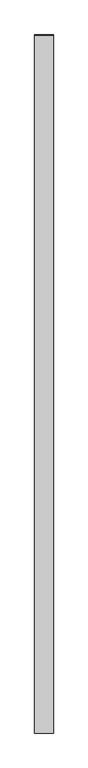
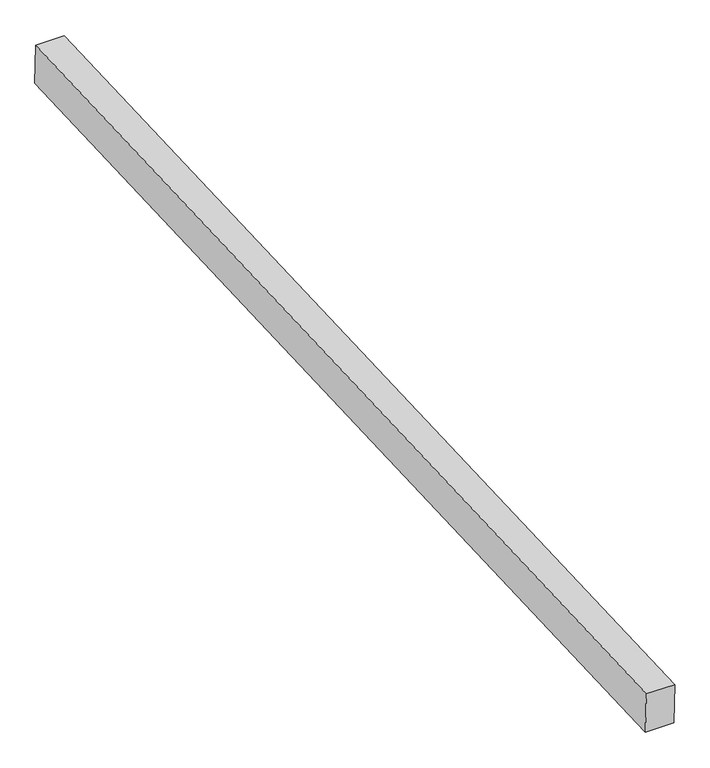
"""IFC4 building model written with IfcOpenShell, lengths in millimetres: proxy geometry, Generic Models 7:Generic Models 1:8:Generic Models 1:8 : Generic Models 7:Generic Models 1:337419:24 : Generic Models 7:Generic Models 1:8:Generic Models 1:8 : Generic Models 7:Generic Models 1:337419:315935."""

import ifcopenshell
import ifcopenshell.guid

model = None  # the IFC model being written
_history = None  # IfcOwnerHistory: only IFC2X3 demands one
_inside = {}  # id of a spatial element -> (the spatial element, [elements in it])
_under = {}  # id of a project, library or spatial element -> (it, [spatial elements below it])
_declared = {}  # id of a project -> (the project, [libraries it declares])
_typed = {}  # id of a type object -> (the type object, [elements of that type])
_made_of = {}  # id of a material, layer set ... -> (it, [elements and type objects made of it])


def new_model(schema):
    """Start an empty IFC model of exactly this schema.

    Asked for "IFC4X3", IfcOpenShell would pick the latest addendum, in which some entities
    have other attributes; the version numbers below select the first issue.
    IFC2X3 requires an IfcOwnerHistory on every rooted entity: one is made here for all.
    """
    global model, _history
    if schema == "IFC4X3":
        model = ifcopenshell.file(schema_version=(4, 3, 0, 0))
    else:
        model = ifcopenshell.file(schema=schema)
    _inside.clear()
    _under.clear()
    _declared.clear()
    _typed.clear()
    _made_of.clear()
    _history = None
    if model.schema == "IFC2X3":
        org = make("IfcOrganization", Name="unknown")
        user = make(
            "IfcPersonAndOrganization",
            ThePerson=make("IfcPerson", FamilyName="unknown"),
            TheOrganization=org,
        )
        app = make(
            "IfcApplication",
            ApplicationDeveloper=org,
            Version="unknown",
            ApplicationFullName="unknown",
            ApplicationIdentifier="unknown",
        )
        _history = make(
            "IfcOwnerHistory",
            OwningUser=user,
            OwningApplication=app,
            ChangeAction="ADDED",
            CreationDate=0,
        )
    return model


def make(cls, **values):
    """One entity of the class cls with the attributes given. An attribute that is None is left unset."""
    return model.create_entity(
        cls, **{name: value for name, value in values.items() if value is not None}
    )


def rooted(cls, **values):
    """An entity with a GlobalId (a new one), such as an element, a storey or a relation."""
    return make(cls, GlobalId=ifcopenshell.guid.new(), OwnerHistory=_history, **values)


def si_unit(unit_type, name, prefix=None):
    """IfcSIUnit, for example si_unit("LENGTHUNIT", "METRE", prefix="MILLI")."""
    return make("IfcSIUnit", UnitType=unit_type, Prefix=prefix, Name=name)


def assignment(units):
    """IfcUnitAssignment: the units of a project."""
    return None if units is None else make("IfcUnitAssignment", Units=units)


def point(xyz):
    """IfcCartesianPoint."""
    return None if xyz is None else make("IfcCartesianPoint", Coordinates=xyz)


def direction(xyz):
    """IfcDirection."""
    return None if xyz is None else make("IfcDirection", DirectionRatios=xyz)


def frame(location, z_axis=None, x_axis=None):
    """IfcAxis2Placement3D, a coordinate frame: its origin and axes. An axis left out is left unset."""
    return make(
        "IfcAxis2Placement3D",
        Location=point(location),
        Axis=direction(z_axis),
        RefDirection=direction(x_axis),
    )


def origin():
    """The frame at (0, 0, 0) with its axes left unset."""
    return frame((0.0, 0.0, 0.0))


def place(relative_to, where):
    """IfcLocalPlacement: puts the frame where relative to a parent placement (None: the world)."""
    return make(
        "IfcLocalPlacement", PlacementRelTo=relative_to, RelativePlacement=where
    )


def context(
    kind, dimensions, precision=None, world=None, true_north=None, identifier=None
):
    """IfcGeometricRepresentationContext, for example the 3D "Model" context."""
    return make(
        "IfcGeometricRepresentationContext",
        ContextIdentifier=identifier,
        ContextType=kind,
        CoordinateSpaceDimension=dimensions,
        Precision=precision,
        WorldCoordinateSystem=world,
        TrueNorth=true_north,
    )


def project(units=None, contexts=None):
    """IfcProject with its units and contexts."""
    return rooted(
        "IfcProject",
        Name="project",
        RepresentationContexts=contexts,
        UnitsInContext=assignment(units),
    )


def spatial(cls, under=None, at=None, **own):
    """A site, building, storey or space (cls), placed at a placement, below another one or the project."""
    s = rooted(cls, ObjectPlacement=at, **own)
    if under is not None:
        _under.setdefault(under.id(), (under, []))[1].append(s)
    return s


def polyline(points):
    """IfcPolyline through the points."""
    return make("IfcPolyline", Points=[point(p) for p in points])


def outline(outer, holes=None, kind="AREA"):
    """IfcArbitraryClosedProfileDef: a profile drawn as a closed curve; with holes, ...WithVoids."""
    if holes is None:
        return make("IfcArbitraryClosedProfileDef", ProfileType=kind, OuterCurve=outer)
    return make(
        "IfcArbitraryProfileDefWithVoids",
        ProfileType=kind,
        OuterCurve=outer,
        InnerCurves=holes,
    )


def extrude(swept, where, along, depth):
    """IfcExtrudedAreaSolid: the profile swept, set in the frame where, extruded along a direction by depth."""
    return make(
        "IfcExtrudedAreaSolid",
        SweptArea=swept,
        Position=where,
        ExtrudedDirection=direction(along),
        Depth=depth,
    )


def shape(context_of_items, identifier, shape_type, items):
    """IfcShapeRepresentation: the items that make up one representation, for example the "Body"."""
    return make(
        "IfcShapeRepresentation",
        ContextOfItems=context_of_items,
        RepresentationIdentifier=identifier,
        RepresentationType=shape_type,
        Items=items,
    )


def source(mapping_origin, context_of_items, identifier, shape_type, items):
    """IfcRepresentationMap: a shape defined once, which mapped items show again and again."""
    return make(
        "IfcRepresentationMap",
        MappingOrigin=mapping_origin,
        MappedRepresentation=shape(context_of_items, identifier, shape_type, items),
    )


def transform(
    local_origin,
    x_axis=None,
    y_axis=None,
    z_axis=None,
    scale=None,
    scale2=None,
    scale3=None,
    uniform=True,
):
    """IfcCartesianTransformationOperator3D, or its non-uniform kind. x_axis, y_axis, z_axis: its Axis1, 2, 3."""
    if uniform:
        return make(
            "IfcCartesianTransformationOperator3D",
            Axis1=direction(x_axis),
            Axis2=direction(y_axis),
            LocalOrigin=point(local_origin),
            Scale=scale,
            Axis3=direction(z_axis),
        )
    return make(
        "IfcCartesianTransformationOperator3DnonUniform",
        Axis1=direction(x_axis),
        Axis2=direction(y_axis),
        LocalOrigin=point(local_origin),
        Scale=scale,
        Axis3=direction(z_axis),
        Scale2=scale2,
        Scale3=scale3,
    )


def mapped(mapping_source, mapping_target):
    """IfcMappedItem: shows the shape of a source again, moved by a transform."""
    return make(
        "IfcMappedItem", MappingSource=mapping_source, MappingTarget=mapping_target
    )


def made_of(thing, what):
    """Note that an element or type object is made of a material, layer set ...; save() writes the relation."""
    if what is not None:
        _made_of.setdefault(what.id(), (what, []))[1].append(thing)
    return thing


def element(
    cls,
    number,
    at=None,
    inside=None,
    cuts=None,
    type_object=None,
    material=None,
    context=None,
    identifier="Body",
    shape_type=None,
    held_by="IfcProductDefinitionShape",
    body=None,
    shapes=None,
    **own,
):
    """One element of the class cls, such as IfcWall. Its Tag is "e" and its number.

    at: its placement. inside: the storey or other place that contains it. cuts: it is an
    opening in that element (IfcRelVoidsElement). A single representation is given by context,
    identifier, shape_type and body (its items); several are given by shapes. held_by: the class
    of the entity that holds the representations. save() writes the other relations.
    """
    e = rooted(cls, Tag="e%d" % number, ObjectPlacement=at, **own)
    if body is not None:
        shapes = [shape(context, identifier, shape_type, body)]
    if shapes is not None:
        e.Representation = make(held_by, Representations=shapes)
    if inside is not None:
        _inside.setdefault(inside.id(), (inside, []))[1].append(e)
    if cuts is not None:
        rooted(
            "IfcRelVoidsElement", RelatingBuildingElement=cuts, RelatedOpeningElement=e
        )
    if type_object is not None:
        _typed.setdefault(type_object.id(), (type_object, []))[1].append(e)
    return made_of(e, material)


def aggregate(whole, parts):
    """IfcRelAggregates: a whole, such as a stair, and the parts it consists of."""
    return rooted("IfcRelAggregates", RelatingObject=whole, RelatedObjects=parts)


def save(model, path):
    """Write the relations noted so far, then the file.

    IfcRelAggregates (storeys below a building ...), IfcRelContainedInSpatialStructure (elements
    in a storey), IfcRelDefinesByType, IfcRelAssociatesMaterial and IfcRelDeclares: one each for
    every whole, place, type object, material and project.
    """
    for whole, parts in _under.values():
        aggregate(whole, parts)
    for where, things in _inside.values():
        rooted(
            "IfcRelContainedInSpatialStructure",
            RelatedElements=things,
            RelatingStructure=where,
        )
    for kind, things in _typed.values():
        rooted("IfcRelDefinesByType", RelatedObjects=things, RelatingType=kind)
    for what, things in _made_of.values():
        rooted("IfcRelAssociatesMaterial", RelatedObjects=things, RelatingMaterial=what)
    for by, libraries in _declared.values():
        rooted("IfcRelDeclares", RelatingContext=by, RelatedDefinitions=libraries)
    model.write(path)


def generic_models_1181b36b(model_context):
    return source(origin(), model_context, "Body", "SweptSolid", [
        extrude(outline(polyline([(-569809.5331551, 8697.9424054), (-564936.6102609, 8900.9808594), (-564929.0433392, 8710.6308549), (-569801.6025364, 8507.607555), (-569809.5331551, 8697.9424054)])), frame((592444.2742243, 0.0, 0.0), z_axis=(1.0, 0.0, 0.0), x_axis=(0.0, 1.0, 0.0)), (0.0, 0.0, 1.0), 130.175),
    ])


if __name__ == "__main__":
    model = new_model("IFC4")
    model_context = context("Model", 3, world=origin())
    ifc_project = project(units=[si_unit("LENGTHUNIT", "METRE", prefix="MILLI")], contexts=[model_context])
    site = spatial("IfcSite", under=ifc_project)
    building = spatial("IfcBuilding", under=site)
    placement = place(None, origin())
    generic_models_shape = generic_models_1181b36b(model_context)
    element("IfcBuildingElementProxy", 1, Name="Generic Models 7:Generic Models 1:8:Generic Models 1:8 : Generic Models 7:Generic Models 1:337419:24 : Generic Models 7:Generic Models 1:8:Generic Models 1:8 : Generic Models 7:Generic Models 1:337419:315935", ObjectType="Generic Models 7:Generic Models 1:8:Generic Models 1:8 : Generic Models 7:Generic Models 1:337419:24 : Generic Models 7:Generic Models 1:8:Generic Models 1:8 : Generic Models 7:Generic Models 1:337419:315935", at=placement, inside=building, context=model_context, shape_type="MappedRepresentation", body=[
        mapped(generic_models_shape, transform((0.0, 0.0, 0.0), x_axis=(1.0, 0.0, 0.0), y_axis=(0.0, 1.0, 0.0), z_axis=(0.0, 0.0, 1.0))),
    ])
    save(model, "model.ifc")

# Revit data of these elements
# Type "Generic Models 7:Generic Models 1:8:Generic Models 1:8 : Generic Models 7:Generic Models 1:337419:24 : Generic Models 7:Generic Models 1:8:Generic Models 1:8 : Generic Models 7:Generic Models 1:337419:315935"
#   NameOverride = "Generic Models 7:Generic Models 1:8:Generic Models 1:8 : Generic Models 7:Generic Models 1:337419:315935"
#   ObjectTypeOverride = "Generic Models 1:8 : Generic Models 7:Generic Models 1:337419"
#   Reference = "Generic Models 1"
#   Tag = "315935"
# Element 1 (IfcBuildingElementProxy, "Generic Models 7:Generic Models 1:8:Generic Models 1:8 : Generic Models 7:Generic Models 1:337419:24 : Generic Models 7:Generic Models 1:8:Generic Models 1:8 : Generic Models 7:Generic Models 1:337419:315935")
#   Materials on its faces: "5 1/8\" X 7 1/2\" EXTERIOR GRADE GLULAM BEAMS (4'- 0 1/4\" O.C.)"
# Materials
#   "5 1/8\" X 7 1/2\" EXTERIOR GRADE GLULAM BEAMS (4'- 0 1/4\" O.C.)": class "Wood", colour RGB 183 134 68, transparency 0, Keynote = "M06181300.01", Description = "Pinus Echinata", Cost = 0
